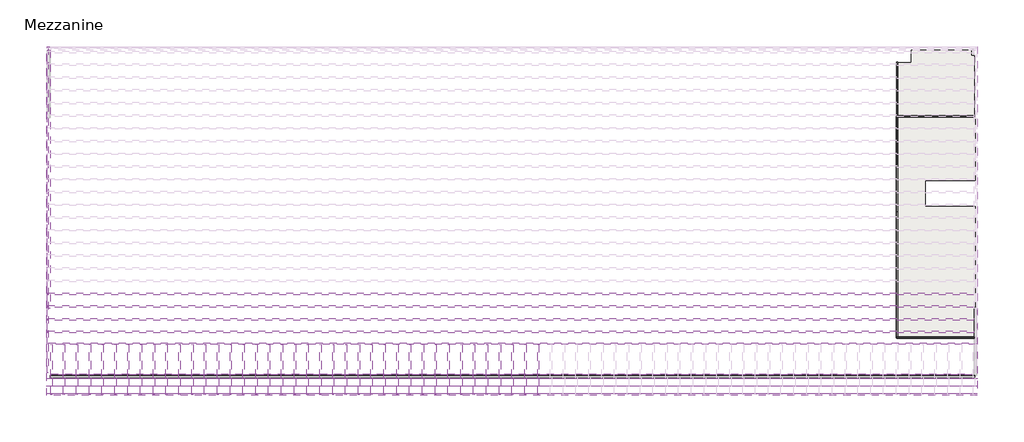
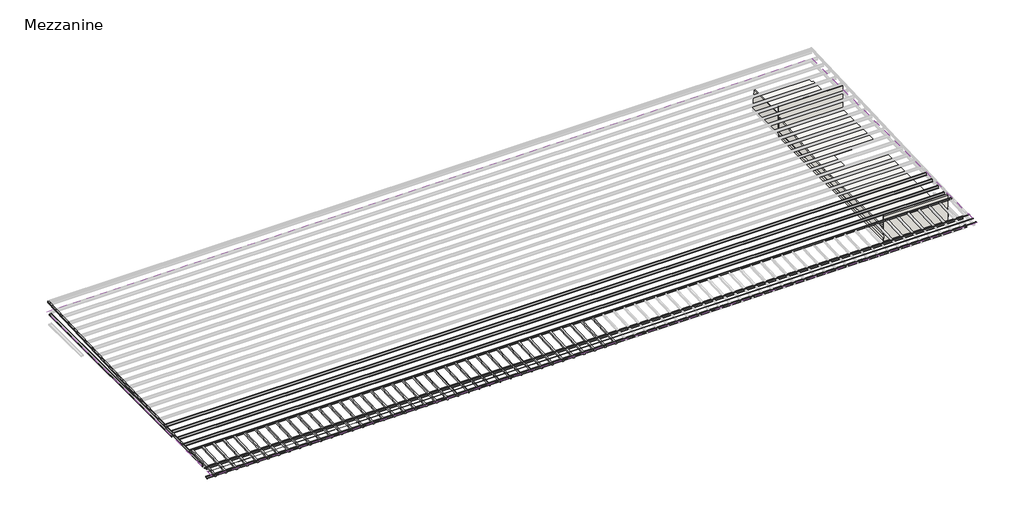
# One storey, part 1 of 2: 51 beams, 4 walls, 2 slabs, 1 roof.
# Revit data of these elements (continued)
# Element 56 (IfcWall, "Generic - Interior - 5\"") (continued)
#   Base Offset = -1' - 0"
#   Unconnected Height = 12' - 0"
#   wall height = 12' - 0"
#   Phase Created = Phase 1
#   Base Constraint = Mezzanine
#   Materials on its faces: "PAINTED GYP. BD.", "Blue, Solid"
# Element 57 (IfcWall, "Generic - Interior - 5\"")
#   built-in parameter 1001111 = -2' - 2 7/32"
#   Top Offset = 0' - 0"
#   Base Offset = -2' - 2 7/32"
#   Unconnected Height = 15' - 5 1/2"
#   wall height = 15' - 5 1/2"
#   Phase Created = Phase 2
#   Base Constraint = Mezzanine
#   Materials on its faces: "PAINTED GYP. BD.", "Blue, Solid"
# Element 58 (IfcWall, "Generic - Interior - 5\"")
#   Top Offset = 0' - 0"
#   Base Offset = 0' - 0"
#   Unconnected Height = 12' - 0"
#   wall height = 12' - 0"
#   Phase Created = Phase 1
#   Base Constraint = Mezzanine
#   Materials on its faces: "PAINTED GYP. BD."
# Materials
#   "Softwood, Lumber": class "Wood", colour RGB 212 179 113, transparency 0, Description = "Pinus Echinata", Cost = 0
#   "1 1/2\" X 1 1/2\" SPLIT-SEAM SQUARE TUBING (~24\" CANTILEVER FROM C.L. OF GLULAM)": class "Metal", colour RGB 199 199 199, transparency 0, Description = "Carbon steel", Cost = 0
#   "Steel ASTM A992": class "Metal", colour RGB 199 199 199, transparency 0, Description = "Structural steel 50ksi", Cost = 0
#   "STRUCTURAL STANDING SEAM SHEET METAL ROOFING - DOUBLE-LOK - COLOR T.B.D.": class "Generic", colour RGB 120 120 120, transparency 0, Keynote = "M09301300.01", Cost = 0
#   "Default Floor": class "Miscellaneous", colour RGB 221 221 221, transparency 0, Cost = 0
#   "PRECAST CONCRETE PLANKS (SEE STRUCT. DWGS)": class "Concrete", colour RGB 198 187 187, transparency 0, Cost = 0
#   "PAINTED GYP. BD.": class "Generic", colour RGB 237 236 233, transparency 0, Description = "Gypsum Wall Board", Cost = 0
#   "Metal Stud Layer": class "Metal", colour RGB 199 199 199, transparency 0, Description = "Light gauge steel framing, thermal air layer", Cost = 0
#   "5 1/2\" X 7 1/2\" EXTERIOR GRADE GLULAM BEAMS": class "Wood", colour RGB 212 179 113, transparency 0, Description = "Pinus Echinata", Cost = 0
#   "CEE' SECTION (8.0x3.5C - SEE STRUCT. DWGS)": class "Metal", colour RGB 137 146 153, transparency 0, Description = "Steel, mill finish", Cost = 0
#   "STRUCTURAL STEEL - SEE STRUCT. DWGS": class "Metal", colour RGB 137 146 153, transparency 0, Description = "Steel, mill finish", Cost = 0
#   "Blue, Solid": class "Paint", colour RGB 67 69 69, transparency 0, Cost = 0
# Space, not placed, phase "Phase 2", upper offset 0' - 0", lower offset 0' - 0"
#   Number = "127"
#   Name = "Electrical Room"
#   Actual Lighting Load per area = 0
#   Actual Power Load per area = 0
#   Sensible Heat Gain per person = 0
#   Specified Lighting Load = 5996.21 (stored number, unit not read)
#   Specified Power Load = 9266.88 (stored number, unit not read)
#   Latent Heat Gain per person = 0
#   Total Heat Gain per person = 0
#   Area per Person = 300 (stored number, unit not read)
#   Number of People = 1.68808 (stored number, unit not read)
#   Lighting Load Units = 0
#   Power Load Units = 0
#   Return Airflow = 0
#   Occupancy Unit = 1
#   Space Type = -1
#   Condition Type = 2
#   Construction Type = none
# Space at (664345.476, -556027.846) mm, phase "Phase 2", upper level "Mezzanine", upper offset 10' - 0", lower offset 0' - 0"
#   Number = "128"
#   Name = "Storage"
#   Actual Lighting Load per area = 0
#   Actual Power Load per area = 0
#   Sensible Heat Gain per person = 0
#   Specified Lighting Load = 19583 (stored number, unit not read)
#   Specified Power Load = 30264.7 (stored number, unit not read)
#   Latent Heat Gain per person = 0
#   Total Heat Gain per person = 0
#   Area per Person = 300 (stored number, unit not read)
#   Number of People = 5.51311 (stored number, unit not read)
#   Lighting Load Units = 0
#   Power Load Units = 0
#   Return Airflow = 0
#   Occupancy Unit = 1
#   Space Type = -1
#   Condition Type = 2
#   Construction Type = none
# Space at (663739.421, -539724.505) mm, phase "Phase 1", upper level "Mezzanine", upper offset 10' - 0", lower offset 0' - 0"
#   Number = "129"
#   Name = "MEZZ. ELEC. ROOM"
#   Occupancy Zone = "Sports Complex"
#   Actual Lighting Load per area = 0
#   Actual Power Load per area = 0
#   Sensible Heat Gain per person = 0
#   Specified Lighting Load = 5844.31 (stored number, unit not read)
#   Specified Power Load = 9032.12 (stored number, unit not read)
#   Latent Heat Gain per person = 0
#   Total Heat Gain per person = 0
#   Area per Person = 300 (stored number, unit not read)
#   Number of People = 1.64532 (stored number, unit not read)
#   Lighting Load Units = 0
#   Power Load Units = 0
#   Return Airflow = 0
#   Occupancy Unit = 1
#   Space Type = -1
#   Condition Type = 2
#   Construction Type = none
# Room at (663678.352, -538266.255) mm, phase "Phase 1", upper level "Mezzanine", upper offset 10' - 0", lower offset 0' - 0"
#   Base Finish = "B1"
#   Floor Finish = "F1"
#   Number = "129"
#   Name = "MEZZ. ELEC. ROOM"
#   North Wall = "W0"
#   South Wall = "W1"
#   West Wall = "W1"
#   East Wall = "W0"
#   Ceiling Finish = "C1"
